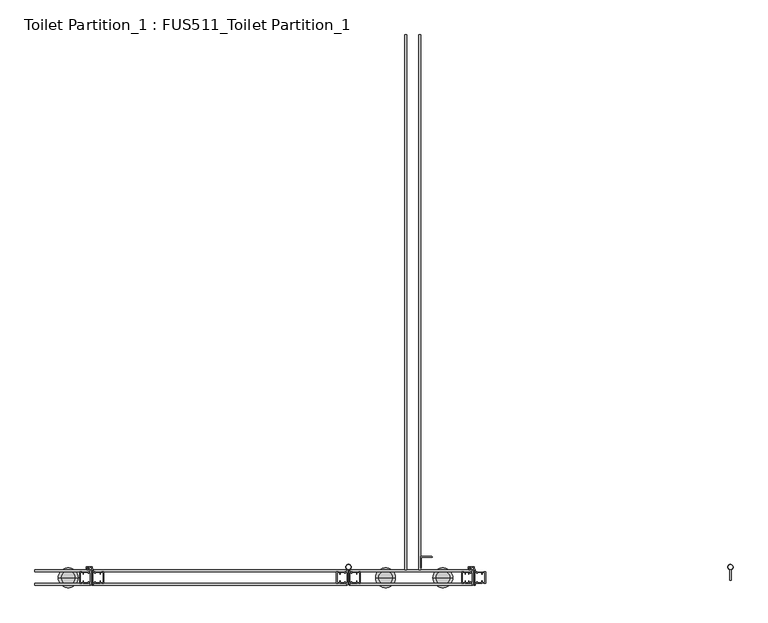
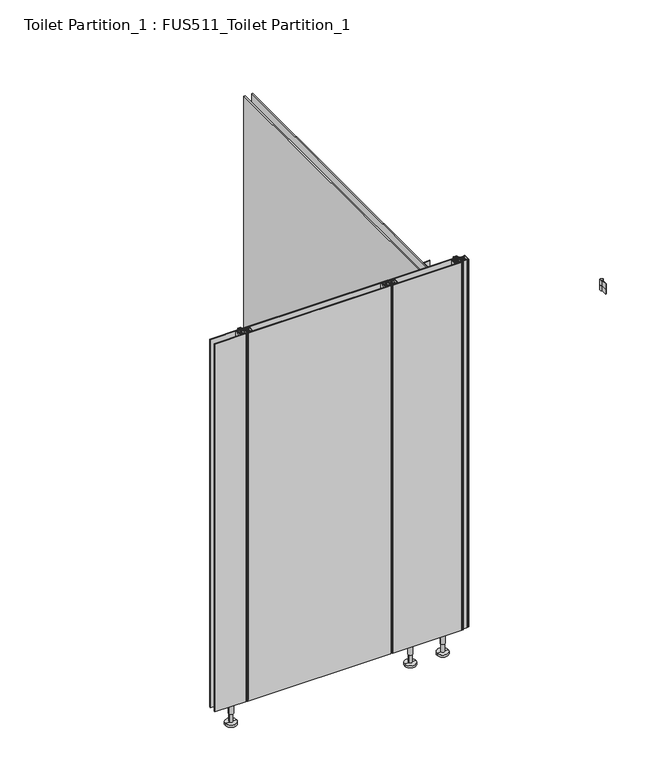
"""IFC4 building model written with IfcOpenShell, lengths in millimetres: furniture geometry, Toilet Partition_1 : FUS511_Toilet Partition_1."""

from ifc_helpers import new_model, si_unit, point, frame, frame_2d, origin, place, context, project, spatial, polyline, circle_curve, trimmed, segment, composite_curve, outline, extrude, source, transform, mapped, element, save
from ifc_brep_helpers import plane_surface, cylinder_surface, advanced_brep


def toilet_partition_1_fus511_toilet_partition_1_6e150948(model_context):
    return source(origin(), model_context, "Body", "SolidModel", [
        extrude(outline(composite_curve([segment(trimmed(circle_curve(frame_2d((-483.6851629, 527.0159753)), 1.0008364), [point((-483.6851629, 528.0168117))], [point((-484.6859993, 527.0159753))], True, "CARTESIAN"), True, "CONTINUOUS"), segment(polyline([(-484.6859993, 527.0159753), (-484.6859993, 499.9933923), (-485.6868357, 499.9933923)]), True, "CONTINUOUS"), segment(trimmed(circle_curve(frame_2d((-485.6868357, 500.9942287)), 1.0008364), [point((-485.6868357, 499.9933923))], [point((-486.6876721, 500.9942287))], False, "CARTESIAN"), True, "CONTINUOUS"), segment(polyline([(-486.6876721, 500.9942287), (-486.6876721, 530.0184846), (-457.6634163, 530.0184846)]), True, "CONTINUOUS"), segment(trimmed(circle_curve(frame_2d((-457.6634163, 529.0176481)), 1.0008364), [point((-457.6634163, 530.0184846))], [point((-456.6625798, 529.0176481))], False, "CARTESIAN"), True, "CONTINUOUS"), segment(polyline([(-456.6625798, 529.0176481), (-456.6625798, 528.0168117), (-483.6851629, 528.0168117)]), True, "CONTINUOUS")], self_intersect=False)), frame((0.0, 0.0, 100.0), z_axis=(0.0, 0.0, 1.0), x_axis=(1.0, 0.0, 0.0)), (0.0, 0.0, 1.0), 1800.0),
        extrude(outline(composite_curve([segment(trimmed(circle_curve(frame_2d((323.7360042, 502.2850056)), 7.0), [point((321.7360042, 495.5768017))], [point((325.7360042, 495.5768017))], False, "CARTESIAN"), True, "CONTINUOUS"), segment(polyline([(325.7360042, 495.5768017), (325.7360042, 467.7850056), (321.7360042, 467.7850056), (321.7360042, 495.5768017)]), True, "CONTINUOUS")], self_intersect=False), holes=[composite_curve([segment(trimmed(circle_curve(frame_2d((323.7360042, 502.2850056)), 6.0), [point((317.7360042, 502.2850056))], [point((329.7360042, 502.2850056))], True, "CARTESIAN"), True, "CONTINUOUS"), segment(trimmed(circle_curve(frame_2d((323.7360042, 502.2850056)), 6.0), [point((329.7360042, 502.2850056))], [point((317.7360042, 502.2850056))], True, "CARTESIAN"), True, "CONTINUOUS")], self_intersect=False)]), frame((0.0, 0.0, 1525.0), z_axis=(0.0, 0.0, 1.0), x_axis=(1.0, 0.0, 0.0)), (0.0, 0.0, 1.0), 25.0),
        extrude(outline(composite_curve([segment(trimmed(circle_curve(frame_2d((323.7360042, 502.2850056)), 7.0), [point((321.7360042, 495.5768017))], [point((325.7360042, 495.5768017))], False, "CARTESIAN"), True, "CONTINUOUS"), segment(polyline([(325.7360042, 495.5768017), (325.7360042, 467.7850056), (321.7360042, 467.7850056), (321.7360042, 495.5768017)]), True, "CONTINUOUS")], self_intersect=False), holes=[composite_curve([segment(trimmed(circle_curve(frame_2d((323.7360042, 502.2850056)), 6.0), [point((317.7360042, 502.2850056))], [point((329.7360042, 502.2850056))], True, "CARTESIAN"), True, "CONTINUOUS"), segment(trimmed(circle_curve(frame_2d((323.7360042, 502.2850056)), 6.0), [point((329.7360042, 502.2850056))], [point((317.7360042, 502.2850056))], True, "CARTESIAN"), True, "CONTINUOUS")], self_intersect=False)]), frame((0.0, 0.0, 1500.0), z_axis=(0.0, 0.0, 1.0), x_axis=(1.0, 0.0, 0.0)), (0.0, 0.0, 1.0), 25.0),
        extrude(outline(composite_curve([segment(trimmed(circle_curve(frame_2d((-675.1953266, 502.2850056)), 7.0), [point((-677.1953266, 495.5768017))], [point((-673.1953266, 495.5768017))], False, "CARTESIAN"), True, "CONTINUOUS"), segment(polyline([(-673.1953266, 495.5768017), (-673.1953266, 467.7850056), (-677.1953266, 467.7850056), (-677.1953266, 495.5768017)]), True, "CONTINUOUS")], self_intersect=False), holes=[composite_curve([segment(trimmed(circle_curve(frame_2d((-675.1953266, 502.2850056)), 6.0), [point((-681.1953266, 502.2850056))], [point((-669.1953266, 502.2850056))], True, "CARTESIAN"), True, "CONTINUOUS"), segment(trimmed(circle_curve(frame_2d((-675.1953266, 502.2850056)), 6.0), [point((-669.1953266, 502.2850056))], [point((-681.1953266, 502.2850056))], True, "CARTESIAN"), True, "CONTINUOUS")], self_intersect=False)]), frame((0.0, 0.0, 1525.0), z_axis=(0.0, 0.0, 1.0), x_axis=(1.0, 0.0, 0.0)), (0.0, 0.0, 1.0), 25.0),
        extrude(outline(composite_curve([segment(trimmed(circle_curve(frame_2d((-675.1953266, 502.2850056)), 7.0), [point((-677.1953266, 495.5768017))], [point((-673.1953266, 495.5768017))], False, "CARTESIAN"), True, "CONTINUOUS"), segment(polyline([(-673.1953266, 495.5768017), (-673.1953266, 467.7850056), (-677.1953266, 467.7850056), (-677.1953266, 495.5768017)]), True, "CONTINUOUS")], self_intersect=False), holes=[composite_curve([segment(trimmed(circle_curve(frame_2d((-675.1953266, 502.2850056)), 6.0), [point((-681.1953266, 502.2850056))], [point((-669.1953266, 502.2850056))], True, "CARTESIAN"), True, "CONTINUOUS"), segment(trimmed(circle_curve(frame_2d((-675.1953266, 502.2850056)), 6.0), [point((-669.1953266, 502.2850056))], [point((-681.1953266, 502.2850056))], True, "CARTESIAN"), True, "CONTINUOUS")], self_intersect=False)]), frame((0.0, 0.0, 1500.0), z_axis=(0.0, 0.0, 1.0), x_axis=(1.0, 0.0, 0.0)), (0.0, 0.0, 1.0), 25.0),
        extrude(outline(composite_curve([segment(trimmed(circle_curve(frame_2d((-675.1953266, 502.2850056)), 7.0), [point((-677.1953266, 495.5768017))], [point((-673.1953266, 495.5768017))], False, "CARTESIAN"), True, "CONTINUOUS"), segment(polyline([(-673.1953266, 495.5768017), (-673.1953266, 467.7850056), (-677.1953266, 467.7850056), (-677.1953266, 495.5768017)]), True, "CONTINUOUS")], self_intersect=False), holes=[composite_curve([segment(trimmed(circle_curve(frame_2d((-675.1953266, 502.2850056)), 6.0), [point((-681.1953266, 502.2850056))], [point((-669.1953266, 502.2850056))], True, "CARTESIAN"), True, "CONTINUOUS"), segment(trimmed(circle_curve(frame_2d((-675.1953266, 502.2850056)), 6.0), [point((-669.1953266, 502.2850056))], [point((-681.1953266, 502.2850056))], True, "CARTESIAN"), True, "CONTINUOUS")], self_intersect=False)]), frame((0.0, 0.0, 525.0), z_axis=(0.0, 0.0, 1.0), x_axis=(1.0, 0.0, 0.0)), (0.0, 0.0, 1.0), 25.0),
        extrude(outline(composite_curve([segment(trimmed(circle_curve(frame_2d((-675.1953266, 502.2850056)), 7.0), [point((-677.1953266, 495.5768017))], [point((-673.1953266, 495.5768017))], False, "CARTESIAN"), True, "CONTINUOUS"), segment(polyline([(-673.1953266, 495.5768017), (-673.1953266, 467.7850056), (-677.1953266, 467.7850056), (-677.1953266, 495.5768017)]), True, "CONTINUOUS")], self_intersect=False), holes=[composite_curve([segment(trimmed(circle_curve(frame_2d((-675.1953266, 502.2850056)), 6.0), [point((-681.1953266, 502.2850056))], [point((-669.1953266, 502.2850056))], True, "CARTESIAN"), True, "CONTINUOUS"), segment(trimmed(circle_curve(frame_2d((-675.1953266, 502.2850056)), 6.0), [point((-669.1953266, 502.2850056))], [point((-681.1953266, 502.2850056))], True, "CARTESIAN"), True, "CONTINUOUS")], self_intersect=False)]), frame((0.0, 0.0, 500.0), z_axis=(0.0, 0.0, 1.0), x_axis=(1.0, 0.0, 0.0)), (0.0, 0.0, 1.0), 25.0),
        extrude(outline(polyline([(-362.0057179, 503.4888254), (-346.2123372, 503.4888254), (-346.2123372, 499.4012527), (-343.7610226, 495.1554513), (-344.9008117, 495.1554513), (-346.2123372, 497.4270801), (-346.2123372, 454.1345106), (-348.1865098, 454.1345106), (-348.1865098, 501.5146528), (-351.8090644, 501.5146528), (-355.8676911, 497.0112968), (-357.0074802, 497.0112968), (-352.9488535, 501.5146528), (-361.0186316, 501.5146528), (-361.0186316, 497.8847941), (-359.6089619, 497.8847941), (-359.6089619, 497.0402783), (-362.0057179, 497.0402783), (-362.0057179, 503.4888254)])), frame((0.0, 0.0, 100.0), z_axis=(0.0, 0.0, 1.0), x_axis=(1.0, 0.0, 0.0)), (0.0, 0.0, 1.0), 1800.0),
        extrude(outline(composite_curve([segment(polyline([(-356.8013826, 495.214347), (-359.8366303, 495.214347)]), True, "CONTINUOUS"), segment(trimmed(circle_curve(frame_2d((-359.8366303, 496.004016)), 0.789669), [point((-359.8366303, 495.214347))], [point((-360.6262994, 496.004016))], False, "CARTESIAN"), True, "CONTINUOUS"), segment(polyline([(-360.6262994, 496.004016), (-360.6262994, 496.8402783), (-359.4784683, 496.8402783)]), True, "CONTINUOUS"), segment(trimmed(circle_curve(frame_2d((-360.1213764, 497.4916495)), 0.9152132), [point((-359.4784683, 496.8402783))], [point((-359.510056, 498.1727534))], True, "CARTESIAN"), True, "CONTINUOUS"), segment(trimmed(circle_curve(frame_2d((-359.2317253, 498.4828563)), 0.4166915), [point((-359.510056, 498.1727534))], [point((-359.3854807, 498.870143))], False, "CARTESIAN"), True, "CONTINUOUS"), segment(trimmed(circle_curve(frame_2d((-358.3136033, 496.1702449)), 2.9048875), [point((-359.3854807, 498.870143))], [point((-357.2177122, 498.8604854))], False, "CARTESIAN"), True, "CONTINUOUS"), segment(trimmed(circle_curve(frame_2d((-357.3679142, 498.4917631)), 0.3981417), [point((-357.2177122, 498.8604854))], [point((-357.1098506, 498.1885801))], False, "CARTESIAN"), True, "CONTINUOUS"), segment(trimmed(circle_curve(frame_2d((-356.5166366, 497.4916495)), 0.9152132), [point((-357.1098506, 498.1885801))], [point((-357.1595447, 496.8402783))], True, "CARTESIAN"), True, "CONTINUOUS"), segment(polyline([(-357.1595447, 496.8402783), (-356.0117136, 496.8402783), (-356.0117136, 496.004016)]), True, "CONTINUOUS"), segment(trimmed(circle_curve(frame_2d((-356.8013826, 496.004016)), 0.789669), [point((-356.0117136, 496.004016))], [point((-356.8013826, 495.214347))], False, "CARTESIAN"), True, "CONTINUOUS")], self_intersect=False)), frame((0.0, 0.0, 100.0), z_axis=(0.0, 0.0, 1.0), x_axis=(1.0, 0.0, 0.0)), (0.0, 0.0, 1.0), 1800.0),
        extrude(outline(polyline([(-1360.9370525, 503.4888254), (-1345.1436718, 503.4888254), (-1345.1436718, 499.4012527), (-1342.6923572, 495.1554513), (-1343.8321463, 495.1554513), (-1345.1436718, 497.4270801), (-1345.1436718, 454.1345106), (-1347.1178444, 454.1345106), (-1347.1178444, 501.5146528), (-1350.740399, 501.5146528), (-1354.7990257, 497.0112968), (-1355.9388148, 497.0112968), (-1351.8801881, 501.5146528), (-1359.9499662, 501.5146528), (-1359.9499662, 497.8847941), (-1358.5402965, 497.8847941), (-1358.5402965, 497.0402783), (-1360.9370525, 497.0402783), (-1360.9370525, 503.4888254)])), frame((0.0, 0.0, 100.0), z_axis=(0.0, 0.0, 1.0), x_axis=(1.0, 0.0, 0.0)), (0.0, 0.0, 1.0), 1800.0),
        extrude(outline(composite_curve([segment(polyline([(-1355.7327172, 495.214347), (-1358.7679649, 495.214347)]), True, "CONTINUOUS"), segment(trimmed(circle_curve(frame_2d((-1358.7679649, 496.004016)), 0.789669), [point((-1358.7679649, 495.214347))], [point((-1359.557634, 496.004016))], False, "CARTESIAN"), True, "CONTINUOUS"), segment(polyline([(-1359.557634, 496.004016), (-1359.557634, 496.8402783), (-1358.4098029, 496.8402783)]), True, "CONTINUOUS"), segment(trimmed(circle_curve(frame_2d((-1359.052711, 497.4916495)), 0.9152132), [point((-1358.4098029, 496.8402783))], [point((-1358.4413906, 498.1727534))], True, "CARTESIAN"), True, "CONTINUOUS"), segment(trimmed(circle_curve(frame_2d((-1358.1630599, 498.4828563)), 0.4166915), [point((-1358.4413906, 498.1727534))], [point((-1358.3168153, 498.870143))], False, "CARTESIAN"), True, "CONTINUOUS"), segment(trimmed(circle_curve(frame_2d((-1357.2449378, 496.1702449)), 2.9048875), [point((-1358.3168153, 498.870143))], [point((-1356.1490468, 498.8604854))], False, "CARTESIAN"), True, "CONTINUOUS"), segment(trimmed(circle_curve(frame_2d((-1356.2992488, 498.4917631)), 0.3981417), [point((-1356.1490468, 498.8604854))], [point((-1356.0411852, 498.1885801))], False, "CARTESIAN"), True, "CONTINUOUS"), segment(trimmed(circle_curve(frame_2d((-1355.4479712, 497.4916495)), 0.9152132), [point((-1356.0411852, 498.1885801))], [point((-1356.0908793, 496.8402783))], True, "CARTESIAN"), True, "CONTINUOUS"), segment(polyline([(-1356.0908793, 496.8402783), (-1354.9430482, 496.8402783), (-1354.9430482, 496.004016)]), True, "CONTINUOUS"), segment(trimmed(circle_curve(frame_2d((-1355.7327172, 496.004016)), 0.789669), [point((-1354.9430482, 496.004016))], [point((-1355.7327172, 495.214347))], False, "CARTESIAN"), True, "CONTINUOUS")], self_intersect=False)), frame((0.0, 0.0, 100.0), z_axis=(0.0, 0.0, 1.0), x_axis=(1.0, 0.0, 0.0)), (0.0, 0.0, 1.0), 1800.0),
        advanced_brep(
        [(-443.912605, 474.714347, 104.1461397), (-412.6687631, 474.714347, 104.1461397), (-412.6687631, 474.714347, 101.0217555), (-443.912605, 474.714347, 101.0217555), (-454.3272189, 474.714347, 0.0), (-402.2541491, 474.714347, 0.0), (-428.290684, 474.714347, 0.0), (-454.3272189, 474.714347, 10.414614), (-402.2541491, 474.714347, 10.414614), (-436.1016445, 474.714347, 10.414614), (-420.4797235, 474.714347, 10.414614), (-436.1016445, 474.714347, 52.0730698), (-420.4797235, 474.714347, 52.0730698), (-438.705298, 474.714347, 52.0730698), (-417.8760701, 474.714347, 52.0730698), (-438.705298, 474.714347, 101.0217555), (-417.8760701, 474.714347, 101.0217555), (-445.9955278, 474.714347, 104.1461397), (-410.5858403, 474.714347, 104.1461397), (-445.9955278, 474.714347, 110.394908), (-410.5858403, 474.714347, 110.394908), (-428.290684, 474.714347, 110.394908)],
        [
            (0, 1, circle_curve(frame((-428.290684, 474.714347, 104.1461397), z_axis=(0.0, 0.0, -1.0), x_axis=(1.0, 0.0, 0.0)), 15.6219209)),
            (1, 2),
            (2, 3, circle_curve(frame((-428.290684, 474.714347, 101.0217555), z_axis=(0.0, 0.0, 1.0), x_axis=(1.0, 0.0, 0.0)), 15.6219209)),
            (3, 0),
            (1, 0, circle_curve(frame((-428.290684, 474.714347, 104.1461397), z_axis=(0.0, 0.0, -1.0), x_axis=(1.0, 0.0, 0.0)), 15.6219209)),
            (3, 2, circle_curve(frame((-428.290684, 474.714347, 101.0217555), z_axis=(0.0, 0.0, 1.0), x_axis=(1.0, 0.0, 0.0)), 15.6219209)),
            (4, 5, circle_curve(frame((-428.290684, 474.714347, 0.0), z_axis=(0.0, 0.0, -1.0), x_axis=(1.0, 0.0, 0.0)), 26.0365349)),
            (5, 6),
            (6, 4),
            (5, 4, circle_curve(frame((-428.290684, 474.714347, 0.0), z_axis=(0.0, 0.0, -1.0), x_axis=(1.0, 0.0, 0.0)), 26.0365349)),
            (7, 8, circle_curve(frame((-428.290684, 474.714347, 10.414614), z_axis=(0.0, 0.0, -1.0), x_axis=(1.0, 0.0, 0.0)), 26.0365349)),
            (8, 5),
            (4, 7),
            (8, 7, circle_curve(frame((-428.290684, 474.714347, 10.414614), z_axis=(0.0, 0.0, -1.0), x_axis=(1.0, 0.0, 0.0)), 26.0365349)),
            (9, 10, circle_curve(frame((-428.290684, 474.714347, 10.414614), z_axis=(0.0, 0.0, -1.0), x_axis=(1.0, 0.0, 0.0)), 7.8109605)),
            (10, 8),
            (7, 9),
            (10, 9, circle_curve(frame((-428.290684, 474.714347, 10.414614), z_axis=(0.0, 0.0, -1.0), x_axis=(1.0, 0.0, 0.0)), 7.8109605)),
            (11, 12, circle_curve(frame((-428.290684, 474.714347, 52.0730698), z_axis=(0.0, 0.0, -1.0), x_axis=(1.0, 0.0, 0.0)), 7.8109605)),
            (12, 10),
            (9, 11),
            (12, 11, circle_curve(frame((-428.290684, 474.714347, 52.0730698), z_axis=(0.0, 0.0, -1.0), x_axis=(1.0, 0.0, 0.0)), 7.8109605)),
            (13, 14, circle_curve(frame((-428.290684, 474.714347, 52.0730698), z_axis=(0.0, 0.0, -1.0), x_axis=(1.0, 0.0, 0.0)), 10.414614)),
            (14, 12),
            (11, 13),
            (14, 13, circle_curve(frame((-428.290684, 474.714347, 52.0730698), z_axis=(0.0, 0.0, -1.0), x_axis=(1.0, 0.0, 0.0)), 10.414614)),
            (15, 16, circle_curve(frame((-428.290684, 474.714347, 101.0217555), z_axis=(0.0, 0.0, -1.0), x_axis=(1.0, 0.0, 0.0)), 10.414614)),
            (16, 14),
            (13, 15),
            (16, 15, circle_curve(frame((-428.290684, 474.714347, 101.0217555), z_axis=(0.0, 0.0, -1.0), x_axis=(1.0, 0.0, 0.0)), 10.414614)),
            (2, 16),
            (15, 3),
            (17, 18, circle_curve(frame((-428.290684, 474.714347, 104.1461397), z_axis=(0.0, 0.0, -1.0), x_axis=(1.0, 0.0, 0.0)), 17.7048437)),
            (18, 1),
            (0, 17),
            (18, 17, circle_curve(frame((-428.290684, 474.714347, 104.1461397), z_axis=(0.0, 0.0, -1.0), x_axis=(1.0, 0.0, 0.0)), 17.7048437)),
            (19, 20, circle_curve(frame((-428.290684, 474.714347, 110.394908), z_axis=(0.0, 0.0, -1.0), x_axis=(1.0, 0.0, 0.0)), 17.7048437)),
            (20, 18),
            (17, 19),
            (20, 19, circle_curve(frame((-428.290684, 474.714347, 110.394908), z_axis=(0.0, 0.0, -1.0), x_axis=(1.0, 0.0, 0.0)), 17.7048437)),
            (21, 20),
            (19, 21),
        ],
        [
            cylinder_surface(frame((-428.290684, 474.714347, 190.0), z_axis=(0.0, 0.0, 1.0), x_axis=(1.0, 0.0, 0.0)), 15.6219209),
            plane_surface(frame((-428.290684, 474.714347, 0.0), z_axis=(0.0, 0.0, -1.0), x_axis=(1.0, 0.0, 0.0))),
            cylinder_surface(frame((-428.290684, 474.714347, 190.0), z_axis=(0.0, 0.0, 1.0), x_axis=(1.0, 0.0, 0.0)), 26.0365349),
            plane_surface(frame((-428.290684, 474.714347, 10.414614), z_axis=(0.0, 0.0, 1.0), x_axis=(1.0, 0.0, 0.0))),
            cylinder_surface(frame((-428.290684, 474.714347, 190.0), z_axis=(0.0, 0.0, 1.0), x_axis=(1.0, 0.0, 0.0)), 7.8109605),
            plane_surface(frame((-428.290684, 474.714347, 52.0730698), z_axis=(0.0, 0.0, -1.0), x_axis=(1.0, 0.0, 0.0))),
            cylinder_surface(frame((-428.290684, 474.714347, 190.0), z_axis=(0.0, 0.0, 1.0), x_axis=(1.0, 0.0, 0.0)), 10.414614),
            plane_surface(frame((-428.290684, 474.714347, 101.0217555), z_axis=(0.0, 0.0, -1.0), x_axis=(1.0, 0.0, 0.0))),
            plane_surface(frame((-428.290684, 474.714347, 104.1461397), z_axis=(0.0, 0.0, -1.0), x_axis=(1.0, 0.0, 0.0))),
            cylinder_surface(frame((-428.290684, 474.714347, 190.0), z_axis=(0.0, 0.0, 1.0), x_axis=(1.0, 0.0, 0.0)), 17.7048437),
            plane_surface(frame((-428.290684, 474.714347, 110.394908), z_axis=(0.0, 0.0, 1.0), x_axis=(1.0, 0.0, 0.0))),
        ],
        [
            (0, [[1, 2, 3, 4]]),
            (0, [[5, -4, 6, -2]]),
            (1, [[7, 8, 9]]),
            (1, [[10, -9, -8]]),
            (2, [[11, 12, -7, 13]]),
            (2, [[14, -13, -10, -12]]),
            (3, [[15, 16, -11, 17]]),
            (3, [[18, -17, -14, -16]]),
            (4, [[19, 20, -15, 21]]),
            (4, [[22, -21, -18, -20]]),
            (5, [[23, 24, -19, 25]]),
            (5, [[26, -25, -22, -24]]),
            (6, [[27, 28, -23, 29]]),
            (6, [[30, -29, -26, -28]]),
            (7, [[-3, 31, -27, 32]]),
            (7, [[-6, -32, -30, -31]]),
            (8, [[33, 34, -1, 35]]),
            (8, [[36, -35, -5, -34]]),
            (9, [[37, 38, -33, 39]]),
            (9, [[40, -39, -36, -38]]),
            (10, [[41, -37, 42]]),
            (10, [[-42, -40, -41]]),
        ],
    ),
        advanced_brep(
        [(-593.912605, 474.714347, 104.1461397), (-562.6687631, 474.714347, 104.1461397), (-562.6687631, 474.714347, 101.0217555), (-593.912605, 474.714347, 101.0217555), (-604.3272189, 474.714347, 0.0), (-552.2541491, 474.714347, 0.0), (-578.290684, 474.714347, 0.0), (-604.3272189, 474.714347, 10.414614), (-552.2541491, 474.714347, 10.414614), (-586.1016445, 474.714347, 10.414614), (-570.4797235, 474.714347, 10.414614), (-586.1016445, 474.714347, 52.0730698), (-570.4797235, 474.714347, 52.0730698), (-588.705298, 474.714347, 52.0730698), (-567.8760701, 474.714347, 52.0730698), (-588.705298, 474.714347, 101.0217555), (-567.8760701, 474.714347, 101.0217555), (-595.9955278, 474.714347, 104.1461397), (-560.5858403, 474.714347, 104.1461397), (-595.9955278, 474.714347, 110.394908), (-560.5858403, 474.714347, 110.394908), (-578.290684, 474.714347, 110.394908)],
        [
            (0, 1, circle_curve(frame((-578.290684, 474.714347, 104.1461397), z_axis=(0.0, 0.0, -1.0), x_axis=(1.0, 0.0, 0.0)), 15.6219209)),
            (1, 2),
            (2, 3, circle_curve(frame((-578.290684, 474.714347, 101.0217555), z_axis=(0.0, 0.0, 1.0), x_axis=(1.0, 0.0, 0.0)), 15.6219209)),
            (3, 0),
            (1, 0, circle_curve(frame((-578.290684, 474.714347, 104.1461397), z_axis=(0.0, 0.0, -1.0), x_axis=(1.0, 0.0, 0.0)), 15.6219209)),
            (3, 2, circle_curve(frame((-578.290684, 474.714347, 101.0217555), z_axis=(0.0, 0.0, 1.0), x_axis=(1.0, 0.0, 0.0)), 15.6219209)),
            (4, 5, circle_curve(frame((-578.290684, 474.714347, 0.0), z_axis=(0.0, 0.0, -1.0), x_axis=(1.0, 0.0, 0.0)), 26.0365349)),
            (5, 6),
            (6, 4),
            (5, 4, circle_curve(frame((-578.290684, 474.714347, 0.0), z_axis=(0.0, 0.0, -1.0), x_axis=(1.0, 0.0, 0.0)), 26.0365349)),
            (7, 8, circle_curve(frame((-578.290684, 474.714347, 10.414614), z_axis=(0.0, 0.0, -1.0), x_axis=(1.0, 0.0, 0.0)), 26.0365349)),
            (8, 5),
            (4, 7),
            (8, 7, circle_curve(frame((-578.290684, 474.714347, 10.414614), z_axis=(0.0, 0.0, -1.0), x_axis=(1.0, 0.0, 0.0)), 26.0365349)),
            (9, 10, circle_curve(frame((-578.290684, 474.714347, 10.414614), z_axis=(0.0, 0.0, -1.0), x_axis=(1.0, 0.0, 0.0)), 7.8109605)),
            (10, 8),
            (7, 9),
            (10, 9, circle_curve(frame((-578.290684, 474.714347, 10.414614), z_axis=(0.0, 0.0, -1.0), x_axis=(1.0, 0.0, 0.0)), 7.8109605)),
            (11, 12, circle_curve(frame((-578.290684, 474.714347, 52.0730698), z_axis=(0.0, 0.0, -1.0), x_axis=(1.0, 0.0, 0.0)), 7.8109605)),
            (12, 10),
            (9, 11),
            (12, 11, circle_curve(frame((-578.290684, 474.714347, 52.0730698), z_axis=(0.0, 0.0, -1.0), x_axis=(1.0, 0.0, 0.0)), 7.8109605)),
            (13, 14, circle_curve(frame((-578.290684, 474.714347, 52.0730698), z_axis=(0.0, 0.0, -1.0), x_axis=(1.0, 0.0, 0.0)), 10.414614)),
            (14, 12),
            (11, 13),
            (14, 13, circle_curve(frame((-578.290684, 474.714347, 52.0730698), z_axis=(0.0, 0.0, -1.0), x_axis=(1.0, 0.0, 0.0)), 10.414614)),
            (15, 16, circle_curve(frame((-578.290684, 474.714347, 101.0217555), z_axis=(0.0, 0.0, -1.0), x_axis=(1.0, 0.0, 0.0)), 10.414614)),
            (16, 14),
            (13, 15),
            (16, 15, circle_curve(frame((-578.290684, 474.714347, 101.0217555), z_axis=(0.0, 0.0, -1.0), x_axis=(1.0, 0.0, 0.0)), 10.414614)),
            (2, 16),
            (15, 3),
            (17, 18, circle_curve(frame((-578.290684, 474.714347, 104.1461397), z_axis=(0.0, 0.0, -1.0), x_axis=(1.0, 0.0, 0.0)), 17.7048437)),
            (18, 1),
            (0, 17),
            (18, 17, circle_curve(frame((-578.290684, 474.714347, 104.1461397), z_axis=(0.0, 0.0, -1.0), x_axis=(1.0, 0.0, 0.0)), 17.7048437)),
            (19, 20, circle_curve(frame((-578.290684, 474.714347, 110.394908), z_axis=(0.0, 0.0, -1.0), x_axis=(1.0, 0.0, 0.0)), 17.7048437)),
            (20, 18),
            (17, 19),
            (20, 19, circle_curve(frame((-578.290684, 474.714347, 110.394908), z_axis=(0.0, 0.0, -1.0), x_axis=(1.0, 0.0, 0.0)), 17.7048437)),
            (21, 20),
            (19, 21),
        ],
        [
            cylinder_surface(frame((-578.290684, 474.714347, 190.0), z_axis=(0.0, 0.0, 1.0), x_axis=(1.0, 0.0, 0.0)), 15.6219209),
            plane_surface(frame((-578.290684, 474.714347, 0.0), z_axis=(0.0, 0.0, -1.0), x_axis=(1.0, 0.0, 0.0))),
            cylinder_surface(frame((-578.290684, 474.714347, 190.0), z_axis=(0.0, 0.0, 1.0), x_axis=(1.0, 0.0, 0.0)), 26.0365349),
            plane_surface(frame((-578.290684, 474.714347, 10.414614), z_axis=(0.0, 0.0, 1.0), x_axis=(1.0, 0.0, 0.0))),
            cylinder_surface(frame((-578.290684, 474.714347, 190.0), z_axis=(0.0, 0.0, 1.0), x_axis=(1.0, 0.0, 0.0)), 7.8109605),
            plane_surface(frame((-578.290684, 474.714347, 52.0730698), z_axis=(0.0, 0.0, -1.0), x_axis=(1.0, 0.0, 0.0))),
            cylinder_surface(frame((-578.290684, 474.714347, 190.0), z_axis=(0.0, 0.0, 1.0), x_axis=(1.0, 0.0, 0.0)), 10.414614),
            plane_surface(frame((-578.290684, 474.714347, 101.0217555), z_axis=(0.0, 0.0, -1.0), x_axis=(1.0, 0.0, 0.0))),
            plane_surface(frame((-578.290684, 474.714347, 104.1461397), z_axis=(0.0, 0.0, -1.0), x_axis=(1.0, 0.0, 0.0))),
            cylinder_surface(frame((-578.290684, 474.714347, 190.0), z_axis=(0.0, 0.0, 1.0), x_axis=(1.0, 0.0, 0.0)), 17.7048437),
            plane_surface(frame((-578.290684, 474.714347, 110.394908), z_axis=(0.0, 0.0, 1.0), x_axis=(1.0, 0.0, 0.0))),
        ],
        [
            (0, [[1, 2, 3, 4]]),
            (0, [[5, -4, 6, -2]]),
            (1, [[7, 8, 9]]),
            (1, [[10, -9, -8]]),
            (2, [[11, 12, -7, 13]]),
            (2, [[14, -13, -10, -12]]),
            (3, [[15, 16, -11, 17]]),
            (3, [[18, -17, -14, -16]]),
            (4, [[19, 20, -15, 21]]),
            (4, [[22, -21, -18, -20]]),
            (5, [[23, 24, -19, 25]]),
            (5, [[26, -25, -22, -24]]),
            (6, [[27, 28, -23, 29]]),
            (6, [[30, -29, -26, -28]]),
            (7, [[-3, 31, -27, 32]]),
            (7, [[-6, -32, -30, -31]]),
            (8, [[33, 34, -1, 35]]),
            (8, [[36, -35, -5, -34]]),
            (9, [[37, 38, -33, 39]]),
            (9, [[40, -39, -36, -38]]),
            (10, [[41, -37, 42]]),
            (10, [[-42, -40, -41]]),
        ],
    ),
        advanced_brep(
        [(-1423.912605, 474.714347, 104.1461397), (-1392.6687631, 474.714347, 104.1461397), (-1392.6687631, 474.714347, 101.0217555), (-1423.912605, 474.714347, 101.0217555), (-1434.3272189, 474.714347, 0.0), (-1382.2541491, 474.714347, 0.0), (-1408.290684, 474.714347, 0.0), (-1434.3272189, 474.714347, 10.414614), (-1382.2541491, 474.714347, 10.414614), (-1416.1016445, 474.714347, 10.414614), (-1400.4797235, 474.714347, 10.414614), (-1416.1016445, 474.714347, 52.0730698), (-1400.4797235, 474.714347, 52.0730698), (-1418.705298, 474.714347, 52.0730698), (-1397.8760701, 474.714347, 52.0730698), (-1418.705298, 474.714347, 101.0217555), (-1397.8760701, 474.714347, 101.0217555), (-1425.9955278, 474.714347, 104.1461397), (-1390.5858403, 474.714347, 104.1461397), (-1425.9955278, 474.714347, 110.394908), (-1390.5858403, 474.714347, 110.394908), (-1408.290684, 474.714347, 110.394908)],
        [
            (0, 1, circle_curve(frame((-1408.290684, 474.714347, 104.1461397), z_axis=(0.0, 0.0, -1.0), x_axis=(1.0, 0.0, 0.0)), 15.6219209)),
            (1, 2),
            (2, 3, circle_curve(frame((-1408.290684, 474.714347, 101.0217555), z_axis=(0.0, 0.0, 1.0), x_axis=(1.0, 0.0, 0.0)), 15.6219209)),
            (3, 0),
            (1, 0, circle_curve(frame((-1408.290684, 474.714347, 104.1461397), z_axis=(0.0, 0.0, -1.0), x_axis=(1.0, 0.0, 0.0)), 15.6219209)),
            (3, 2, circle_curve(frame((-1408.290684, 474.714347, 101.0217555), z_axis=(0.0, 0.0, 1.0), x_axis=(1.0, 0.0, 0.0)), 15.6219209)),
            (4, 5, circle_curve(frame((-1408.290684, 474.714347, 0.0), z_axis=(0.0, 0.0, -1.0), x_axis=(1.0, 0.0, 0.0)), 26.0365349)),
            (5, 6),
            (6, 4),
            (5, 4, circle_curve(frame((-1408.290684, 474.714347, 0.0), z_axis=(0.0, 0.0, -1.0), x_axis=(1.0, 0.0, 0.0)), 26.0365349)),
            (7, 8, circle_curve(frame((-1408.290684, 474.714347, 10.414614), z_axis=(0.0, 0.0, -1.0), x_axis=(1.0, 0.0, 0.0)), 26.0365349)),
            (8, 5),
            (4, 7),
            (8, 7, circle_curve(frame((-1408.290684, 474.714347, 10.414614), z_axis=(0.0, 0.0, -1.0), x_axis=(1.0, 0.0, 0.0)), 26.0365349)),
            (9, 10, circle_curve(frame((-1408.290684, 474.714347, 10.414614), z_axis=(0.0, 0.0, -1.0), x_axis=(1.0, 0.0, 0.0)), 7.8109605)),
            (10, 8),
            (7, 9),
            (10, 9, circle_curve(frame((-1408.290684, 474.714347, 10.414614), z_axis=(0.0, 0.0, -1.0), x_axis=(1.0, 0.0, 0.0)), 7.8109605)),
            (11, 12, circle_curve(frame((-1408.290684, 474.714347, 52.0730698), z_axis=(0.0, 0.0, -1.0), x_axis=(1.0, 0.0, 0.0)), 7.8109605)),
            (12, 10),
            (9, 11),
            (12, 11, circle_curve(frame((-1408.290684, 474.714347, 52.0730698), z_axis=(0.0, 0.0, -1.0), x_axis=(1.0, 0.0, 0.0)), 7.8109605)),
            (13, 14, circle_curve(frame((-1408.290684, 474.714347, 52.0730698), z_axis=(0.0, 0.0, -1.0), x_axis=(1.0, 0.0, 0.0)), 10.414614)),
            (14, 12),
            (11, 13),
            (14, 13, circle_curve(frame((-1408.290684, 474.714347, 52.0730698), z_axis=(0.0, 0.0, -1.0), x_axis=(1.0, 0.0, 0.0)), 10.414614)),
            (15, 16, circle_curve(frame((-1408.290684, 474.714347, 101.0217555), z_axis=(0.0, 0.0, -1.0), x_axis=(1.0, 0.0, 0.0)), 10.414614)),
            (16, 14),
            (13, 15),
            (16, 15, circle_curve(frame((-1408.290684, 474.714347, 101.0217555), z_axis=(0.0, 0.0, -1.0), x_axis=(1.0, 0.0, 0.0)), 10.414614)),
            (2, 16),
            (15, 3),
            (17, 18, circle_curve(frame((-1408.290684, 474.714347, 104.1461397), z_axis=(0.0, 0.0, -1.0), x_axis=(1.0, 0.0, 0.0)), 17.7048437)),
            (18, 1),
            (0, 17),
            (18, 17, circle_curve(frame((-1408.290684, 474.714347, 104.1461397), z_axis=(0.0, 0.0, -1.0), x_axis=(1.0, 0.0, 0.0)), 17.7048437)),
            (19, 20, circle_curve(frame((-1408.290684, 474.714347, 110.394908), z_axis=(0.0, 0.0, -1.0), x_axis=(1.0, 0.0, 0.0)), 17.7048437)),
            (20, 18),
            (17, 19),
            (20, 19, circle_curve(frame((-1408.290684, 474.714347, 110.394908), z_axis=(0.0, 0.0, -1.0), x_axis=(1.0, 0.0, 0.0)), 17.7048437)),
            (21, 20),
            (19, 21),
        ],
        [
            cylinder_surface(frame((-1408.290684, 474.714347, 190.0), z_axis=(0.0, 0.0, 1.0), x_axis=(1.0, 0.0, 0.0)), 15.6219209),
            plane_surface(frame((-1408.290684, 474.714347, 0.0), z_axis=(0.0, 0.0, -1.0), x_axis=(1.0, 0.0, 0.0))),
            cylinder_surface(frame((-1408.290684, 474.714347, 190.0), z_axis=(0.0, 0.0, 1.0), x_axis=(1.0, 0.0, 0.0)), 26.0365349),
            plane_surface(frame((-1408.290684, 474.714347, 10.414614), z_axis=(0.0, 0.0, 1.0), x_axis=(1.0, 0.0, 0.0))),
            cylinder_surface(frame((-1408.290684, 474.714347, 190.0), z_axis=(0.0, 0.0, 1.0), x_axis=(1.0, 0.0, 0.0)), 7.8109605),
            plane_surface(frame((-1408.290684, 474.714347, 52.0730698), z_axis=(0.0, 0.0, -1.0), x_axis=(1.0, 0.0, 0.0))),
            cylinder_surface(frame((-1408.290684, 474.714347, 190.0), z_axis=(0.0, 0.0, 1.0), x_axis=(1.0, 0.0, 0.0)), 10.414614),
            plane_surface(frame((-1408.290684, 474.714347, 101.0217555), z_axis=(0.0, 0.0, -1.0), x_axis=(1.0, 0.0, 0.0))),
            plane_surface(frame((-1408.290684, 474.714347, 104.1461397), z_axis=(0.0, 0.0, -1.0), x_axis=(1.0, 0.0, 0.0))),
            cylinder_surface(frame((-1408.290684, 474.714347, 190.0), z_axis=(0.0, 0.0, 1.0), x_axis=(1.0, 0.0, 0.0)), 17.7048437),
            plane_surface(frame((-1408.290684, 474.714347, 110.394908), z_axis=(0.0, 0.0, 1.0), x_axis=(1.0, 0.0, 0.0))),
        ],
        [
            (0, [[1, 2, 3, 4]]),
            (0, [[5, -4, 6, -2]]),
            (1, [[7, 8, 9]]),
            (1, [[10, -9, -8]]),
            (2, [[11, 12, -7, 13]]),
            (2, [[14, -13, -10, -12]]),
            (3, [[15, 16, -11, 17]]),
            (3, [[18, -17, -14, -16]]),
            (4, [[19, 20, -15, 21]]),
            (4, [[22, -21, -18, -20]]),
            (5, [[23, 24, -19, 25]]),
            (5, [[26, -25, -22, -24]]),
            (6, [[27, 28, -23, 29]]),
            (6, [[30, -29, -26, -28]]),
            (7, [[-3, 31, -27, 32]]),
            (7, [[-6, -32, -30, -31]]),
            (8, [[33, 34, -1, 35]]),
            (8, [[36, -35, -5, -34]]),
            (9, [[37, 38, -33, 39]]),
            (9, [[40, -39, -36, -38]]),
            (10, [[41, -37, 42]]),
            (10, [[-42, -40, -41]]),
        ],
    ),
        extrude(outline(polyline([(-486.6876721, 495.214347), (-491.6876721, 495.214347), (-491.6876721, 1895.214347), (-486.6876721, 1895.214347), (-486.6876721, 495.214347)])), frame((0.0, 0.0, 100.0), z_axis=(0.0, 0.0, 1.0), x_axis=(1.0, 0.0, 0.0)), (0.0, 0.0, 1.0), 1800.0),
        extrude(outline(polyline([(-522.6876721, 495.214347), (-527.6876721, 495.214347), (-527.6876721, 1895.214347), (-522.6876721, 1895.214347), (-522.6876721, 495.214347)])), frame((0.0, 0.0, 100.0), z_axis=(0.0, 0.0, 1.0), x_axis=(1.0, 0.0, 0.0)), (0.0, 0.0, 1.0), 1800.0),
        extrude(outline(composite_curve([segment(polyline([(-1378.0265961, 489.5206414), (-1373.0911646, 489.5206414), (-1373.0911646, 488.5335551), (-1369.1428194, 488.5335551), (-1355.5703828, 489.5206414)]), True, "CONTINUOUS"), segment(trimmed(circle_curve(frame_2d((-1355.3236113, 488.5648992)), 0.9870863), [point((-1355.5703828, 489.5206414))], [point((-1355.0768397, 489.5206414))], True, "CARTESIAN"), True, "CONTINUOUS"), segment(polyline([(-1355.0768397, 489.5206414), (-1350.3881798, 489.5206414), (-1350.3881798, 494.4560729), (-1349.4010935, 494.4560729)]), True, "CONTINUOUS"), segment(trimmed(circle_curve(frame_2d((-1349.4010935, 493.4689866)), 0.9870863), [point((-1349.4010935, 494.4560729))], [point((-1348.4140072, 493.4689866))], False, "CARTESIAN"), True, "CONTINUOUS"), segment(polyline([(-1348.4140072, 493.4689866), (-1348.4140072, 455.9597074)]), True, "CONTINUOUS"), segment(trimmed(circle_curve(frame_2d((-1349.4010935, 455.9597074)), 0.9870863), [point((-1348.4140072, 455.9597074))], [point((-1349.4010935, 454.9726211))], False, "CARTESIAN"), True, "CONTINUOUS"), segment(polyline([(-1349.4010935, 454.9726211), (-1350.3881798, 454.9726211), (-1350.3881798, 459.9080525), (-1355.0768397, 459.9080525)]), True, "CONTINUOUS"), segment(trimmed(circle_curve(frame_2d((-1355.3236113, 460.8637947)), 0.9870863), [point((-1355.0768397, 459.9080525))], [point((-1355.5703828, 459.9080525))], True, "CARTESIAN"), True, "CONTINUOUS"), segment(polyline([(-1355.5703828, 459.9080525), (-1369.1428194, 459.9080525), (-1369.1428194, 460.8951388), (-1373.0911646, 460.8951388), (-1373.0911646, 459.9080525), (-1378.0265961, 459.9080525), (-1378.0265961, 489.5206414)]), True, "CONTINUOUS")], self_intersect=False), holes=[polyline([(-1375.0653372, 486.5593825), (-1375.0653372, 462.8693114), (-1370.1299057, 462.8693114), (-1370.1299057, 467.8047429), (-1367.1686468, 467.8047429), (-1367.1686468, 462.8693114), (-1360.2590427, 462.8693114), (-1360.2590427, 467.3111998), (-1358.7784133, 467.3111998), (-1358.7784133, 462.8693114), (-1357.0510123, 462.8693114), (-1357.0510123, 464.843484), (-1353.1026671, 464.843484), (-1353.1026671, 462.8693114), (-1351.3752661, 462.8693114), (-1351.3752661, 486.5593825), (-1353.1026671, 486.5593825), (-1353.1026671, 484.5852099), (-1357.0510123, 484.5852099), (-1357.0510123, 486.5593825), (-1358.7784133, 486.5593825), (-1358.7784133, 482.1174942), (-1360.2590427, 482.1174942), (-1360.2590427, 486.5593825), (-1367.1686468, 486.5593825), (-1367.1686468, 481.623951), (-1370.1299057, 481.623951), (-1370.1299057, 486.5593825), (-1375.0653372, 486.5593825)])]), frame((0.0, 0.0, 100.0), z_axis=(0.0, 0.0, 1.0), x_axis=(1.0, 0.0, 0.0)), (0.0, 0.0, 1.0), 1800.0),
        extrude(outline(polyline([(-1495.3881798, 454.214347), (-1495.3881798, 459.214347), (-1350.3881798, 459.214347), (-1350.3881798, 454.214347), (-1495.3881798, 454.214347)])), frame((0.0, 0.0, 100.0), z_axis=(0.0, 0.0, 1.0), x_axis=(1.0, 0.0, 0.0)), (0.0, 0.0, 1.0), 1800.0),
        extrude(outline(polyline([(-1495.3881798, 490.214347), (-1495.3881798, 495.214347), (-1350.3881798, 495.214347), (-1350.3881798, 490.214347), (-1495.3881798, 490.214347)])), frame((0.0, 0.0, 100.0), z_axis=(0.0, 0.0, 1.0), x_axis=(1.0, 0.0, 0.0)), (0.0, 0.0, 1.0), 1800.0),
        extrude(outline(composite_curve([segment(polyline([(-1315.5310829, 489.5206414), (-1315.5310829, 459.9080525), (-1320.4665144, 459.9080525), (-1320.4665144, 460.8951388), (-1324.4148596, 460.8951388), (-1324.4148596, 459.9080525), (-1337.9872961, 459.9080525)]), True, "CONTINUOUS"), segment(trimmed(circle_curve(frame_2d((-1338.2340677, 460.8637947)), 0.9870863), [point((-1337.9872961, 459.9080525))], [point((-1338.4808393, 459.9080525))], True, "CARTESIAN"), True, "CONTINUOUS"), segment(polyline([(-1338.4808393, 459.9080525), (-1343.1694992, 459.9080525), (-1343.1694992, 454.9726211), (-1344.1565855, 454.9726211)]), True, "CONTINUOUS"), segment(trimmed(circle_curve(frame_2d((-1344.1565855, 455.9597074)), 0.9870863), [point((-1344.1565855, 454.9726211))], [point((-1345.1436718, 455.9597074))], False, "CARTESIAN"), True, "CONTINUOUS"), segment(polyline([(-1345.1436718, 455.9597074), (-1345.1436718, 493.4689866)]), True, "CONTINUOUS"), segment(trimmed(circle_curve(frame_2d((-1344.1565855, 493.4689866)), 0.9870863), [point((-1345.1436718, 493.4689866))], [point((-1344.1565855, 494.4560729))], False, "CARTESIAN"), True, "CONTINUOUS"), segment(polyline([(-1344.1565855, 494.4560729), (-1343.1694992, 494.4560729), (-1343.1694992, 489.5206414), (-1338.4808393, 489.5206414)]), True, "CONTINUOUS"), segment(trimmed(circle_curve(frame_2d((-1338.2340677, 488.5648992)), 0.9870863), [point((-1338.4808393, 489.5206414))], [point((-1337.9872961, 489.5206414))], True, "CARTESIAN"), True, "CONTINUOUS"), segment(polyline([(-1337.9872961, 489.5206414), (-1324.4148596, 488.5335551), (-1320.4665144, 488.5335551), (-1320.4665144, 489.5206414), (-1315.5310829, 489.5206414)]), True, "CONTINUOUS")], self_intersect=False), holes=[polyline([(-1318.4923418, 486.5593825), (-1323.4277733, 486.5593825), (-1323.4277733, 481.623951), (-1326.3890322, 481.623951), (-1326.3890322, 486.5593825), (-1333.2986362, 486.5593825), (-1333.2986362, 482.1174942), (-1334.7792657, 482.1174942), (-1334.7792657, 486.5593825), (-1336.5066667, 486.5593825), (-1336.5066667, 484.5852099), (-1340.4550119, 484.5852099), (-1340.4550119, 486.5593825), (-1342.1824129, 486.5593825), (-1342.1824129, 462.8693114), (-1340.4550119, 462.8693114), (-1340.4550119, 464.843484), (-1336.5066667, 464.843484), (-1336.5066667, 462.8693114), (-1334.7792657, 462.8693114), (-1334.7792657, 467.3111998), (-1333.2986362, 467.3111998), (-1333.2986362, 462.8693114), (-1326.3890322, 462.8693114), (-1326.3890322, 467.8047429), (-1323.4277733, 467.8047429), (-1323.4277733, 462.8693114), (-1318.4923418, 462.8693114), (-1318.4923418, 486.5593825)])]), frame((0.0, 0.0, 100.0), z_axis=(0.0, 0.0, 1.0), x_axis=(1.0, 0.0, 0.0)), (0.0, 0.0, 1.0), 1800.0),
        extrude(outline(composite_curve([segment(polyline([(-706.8079154, 489.5206414), (-701.872484, 489.5206414), (-701.872484, 488.5335551), (-697.9241388, 488.5335551), (-684.3517022, 489.5206414)]), True, "CONTINUOUS"), segment(trimmed(circle_curve(frame_2d((-684.1049306, 488.5648992)), 0.9870863), [point((-684.3517022, 489.5206414))], [point((-683.8581591, 489.5206414))], True, "CARTESIAN"), True, "CONTINUOUS"), segment(polyline([(-683.8581591, 489.5206414), (-679.1694992, 489.5206414), (-679.1694992, 494.4560729), (-678.1824129, 494.4560729)]), True, "CONTINUOUS"), segment(trimmed(circle_curve(frame_2d((-678.1824129, 493.4689866)), 0.9870863), [point((-678.1824129, 494.4560729))], [point((-677.1953266, 493.4689866))], False, "CARTESIAN"), True, "CONTINUOUS"), segment(polyline([(-677.1953266, 493.4689866), (-677.1953266, 455.9597074)]), True, "CONTINUOUS"), segment(trimmed(circle_curve(frame_2d((-678.1824129, 455.9597074)), 0.9870863), [point((-677.1953266, 455.9597074))], [point((-678.1824129, 454.9726211))], False, "CARTESIAN"), True, "CONTINUOUS"), segment(polyline([(-678.1824129, 454.9726211), (-679.1694992, 454.9726211), (-679.1694992, 459.9080525), (-683.8581591, 459.9080525)]), True, "CONTINUOUS"), segment(trimmed(circle_curve(frame_2d((-684.1049306, 460.8637947)), 0.9870863), [point((-683.8581591, 459.9080525))], [point((-684.3517022, 459.9080525))], True, "CARTESIAN"), True, "CONTINUOUS"), segment(polyline([(-684.3517022, 459.9080525), (-697.9241388, 459.9080525), (-697.9241388, 460.8951388), (-701.872484, 460.8951388), (-701.872484, 459.9080525), (-706.8079154, 459.9080525), (-706.8079154, 489.5206414)]), True, "CONTINUOUS")], self_intersect=False), holes=[polyline([(-703.8466566, 486.5593825), (-703.8466566, 462.8693114), (-698.9112251, 462.8693114), (-698.9112251, 467.8047429), (-695.9499662, 467.8047429), (-695.9499662, 462.8693114), (-689.0403621, 462.8693114), (-689.0403621, 467.3111998), (-687.5597327, 467.3111998), (-687.5597327, 462.8693114), (-685.8323317, 462.8693114), (-685.8323317, 464.843484), (-681.8839865, 464.843484), (-681.8839865, 462.8693114), (-680.1565855, 462.8693114), (-680.1565855, 486.5593825), (-681.8839865, 486.5593825), (-681.8839865, 484.5852099), (-685.8323317, 484.5852099), (-685.8323317, 486.5593825), (-687.5597327, 486.5593825), (-687.5597327, 482.1174942), (-689.0403621, 482.1174942), (-689.0403621, 486.5593825), (-695.9499662, 486.5593825), (-695.9499662, 481.623951), (-698.9112251, 481.623951), (-698.9112251, 486.5593825), (-703.8466566, 486.5593825)])]), frame((0.0, 0.0, 100.0), z_axis=(0.0, 0.0, 1.0), x_axis=(1.0, 0.0, 0.0)), (0.0, 0.0, 1.0), 1800.0),
        extrude(outline(polyline([(-1343.1694992, 454.214347), (-1343.1694992, 459.214347), (-679.1694992, 459.214347), (-679.1694992, 454.214347), (-1343.1694992, 454.214347)])), frame((0.0, 0.0, 100.0), z_axis=(0.0, 0.0, 1.0), x_axis=(1.0, 0.0, 0.0)), (0.0, 0.0, 1.0), 1800.0),
        extrude(outline(polyline([(-1343.1694992, 490.214347), (-1343.1694992, 495.214347), (-679.1694992, 495.214347), (-679.1694992, 490.214347), (-1343.1694992, 490.214347)])), frame((0.0, 0.0, 100.0), z_axis=(0.0, 0.0, 1.0), x_axis=(1.0, 0.0, 0.0)), (0.0, 0.0, 1.0), 1800.0),
        extrude(outline(composite_curve([segment(polyline([(-643.818433, 489.5206414), (-643.818433, 459.9080525), (-648.7538644, 459.9080525), (-648.7538644, 460.8951388), (-652.7022096, 460.8951388), (-652.7022096, 459.9080525), (-666.2746462, 459.9080525)]), True, "CONTINUOUS"), segment(trimmed(circle_curve(frame_2d((-666.5214178, 460.8637947)), 0.9870863), [point((-666.2746462, 459.9080525))], [point((-666.7681893, 459.9080525))], True, "CARTESIAN"), True, "CONTINUOUS"), segment(polyline([(-666.7681893, 459.9080525), (-671.4568492, 459.9080525), (-671.4568492, 454.9726211), (-672.4439355, 454.9726211)]), True, "CONTINUOUS"), segment(trimmed(circle_curve(frame_2d((-672.4439355, 455.9597074)), 0.9870863), [point((-672.4439355, 454.9726211))], [point((-673.4310218, 455.9597074))], False, "CARTESIAN"), True, "CONTINUOUS"), segment(polyline([(-673.4310218, 455.9597074), (-673.4310218, 493.4689866)]), True, "CONTINUOUS"), segment(trimmed(circle_curve(frame_2d((-672.4439355, 493.4689866)), 0.9870863), [point((-673.4310218, 493.4689866))], [point((-672.4439355, 494.4560729))], False, "CARTESIAN"), True, "CONTINUOUS"), segment(polyline([(-672.4439355, 494.4560729), (-671.4568492, 494.4560729), (-671.4568492, 489.5206414), (-666.7681893, 489.5206414)]), True, "CONTINUOUS"), segment(trimmed(circle_curve(frame_2d((-666.5214178, 488.5648992)), 0.9870863), [point((-666.7681893, 489.5206414))], [point((-666.2746462, 489.5206414))], True, "CARTESIAN"), True, "CONTINUOUS"), segment(polyline([(-666.2746462, 489.5206414), (-652.7022096, 488.5335551), (-648.7538644, 488.5335551), (-648.7538644, 489.5206414), (-643.818433, 489.5206414)]), True, "CONTINUOUS")], self_intersect=False), holes=[polyline([(-646.7796918, 486.5593825), (-651.7151233, 486.5593825), (-651.7151233, 481.623951), (-654.6763822, 481.623951), (-654.6763822, 486.5593825), (-661.5859863, 486.5593825), (-661.5859863, 482.1174942), (-663.0666157, 482.1174942), (-663.0666157, 486.5593825), (-664.7940167, 486.5593825), (-664.7940167, 484.5852099), (-668.7423619, 484.5852099), (-668.7423619, 486.5593825), (-670.4697629, 486.5593825), (-670.4697629, 462.8693114), (-668.7423619, 462.8693114), (-668.7423619, 464.843484), (-664.7940167, 464.843484), (-664.7940167, 462.8693114), (-663.0666157, 462.8693114), (-663.0666157, 467.3111998), (-661.5859863, 467.3111998), (-661.5859863, 462.8693114), (-654.6763822, 462.8693114), (-654.6763822, 467.8047429), (-651.7151233, 467.8047429), (-651.7151233, 462.8693114), (-646.7796918, 462.8693114), (-646.7796918, 486.5593825)])]), frame((0.0, 0.0, 100.0), z_axis=(0.0, 0.0, 1.0), x_axis=(1.0, 0.0, 0.0)), (0.0, 0.0, 1.0), 1800.0),
        extrude(outline(composite_curve([segment(polyline([(-379.0952655, 489.5206414), (-374.159834, 489.5206414), (-374.159834, 488.5335551), (-370.2114888, 488.5335551), (-356.6390523, 489.5206414)]), True, "CONTINUOUS"), segment(trimmed(circle_curve(frame_2d((-356.3922807, 488.5648992)), 0.9870863), [point((-356.6390523, 489.5206414))], [point((-356.1455091, 489.5206414))], True, "CARTESIAN"), True, "CONTINUOUS"), segment(polyline([(-356.1455091, 489.5206414), (-351.4568492, 489.5206414), (-351.4568492, 494.4560729), (-350.4697629, 494.4560729)]), True, "CONTINUOUS"), segment(trimmed(circle_curve(frame_2d((-350.4697629, 493.4689866)), 0.9870863), [point((-350.4697629, 494.4560729))], [point((-349.4826766, 493.4689866))], False, "CARTESIAN"), True, "CONTINUOUS"), segment(polyline([(-349.4826766, 493.4689866), (-349.4826766, 455.9597074)]), True, "CONTINUOUS"), segment(trimmed(circle_curve(frame_2d((-350.4697629, 455.9597074)), 0.9870863), [point((-349.4826766, 455.9597074))], [point((-350.4697629, 454.9726211))], False, "CARTESIAN"), True, "CONTINUOUS"), segment(polyline([(-350.4697629, 454.9726211), (-351.4568492, 454.9726211), (-351.4568492, 459.9080525), (-356.1455091, 459.9080525)]), True, "CONTINUOUS"), segment(trimmed(circle_curve(frame_2d((-356.3922807, 460.8637947)), 0.9870863), [point((-356.1455091, 459.9080525))], [point((-356.6390523, 459.9080525))], True, "CARTESIAN"), True, "CONTINUOUS"), segment(polyline([(-356.6390523, 459.9080525), (-370.2114888, 459.9080525), (-370.2114888, 460.8951388), (-374.159834, 460.8951388), (-374.159834, 459.9080525), (-379.0952655, 459.9080525), (-379.0952655, 489.5206414)]), True, "CONTINUOUS")], self_intersect=False), holes=[polyline([(-376.1340066, 486.5593825), (-376.1340066, 462.8693114), (-371.1985751, 462.8693114), (-371.1985751, 467.8047429), (-368.2373162, 467.8047429), (-368.2373162, 462.8693114), (-361.3277122, 462.8693114), (-361.3277122, 467.3111998), (-359.8470827, 467.3111998), (-359.8470827, 462.8693114), (-358.1196817, 462.8693114), (-358.1196817, 464.843484), (-354.1713365, 464.843484), (-354.1713365, 462.8693114), (-352.4439355, 462.8693114), (-352.4439355, 486.5593825), (-354.1713365, 486.5593825), (-354.1713365, 484.5852099), (-358.1196817, 484.5852099), (-358.1196817, 486.5593825), (-359.8470827, 486.5593825), (-359.8470827, 482.1174942), (-361.3277122, 482.1174942), (-361.3277122, 486.5593825), (-368.2373162, 486.5593825), (-368.2373162, 481.623951), (-371.1985751, 481.623951), (-371.1985751, 486.5593825), (-376.1340066, 486.5593825)])]), frame((0.0, 0.0, 100.0), z_axis=(0.0, 0.0, 1.0), x_axis=(1.0, 0.0, 0.0)), (0.0, 0.0, 1.0), 1800.0),
        extrude(outline(polyline([(-671.4568492, 454.214347), (-671.4568492, 459.214347), (-351.4568492, 459.214347), (-351.4568492, 454.214347), (-671.4568492, 454.214347)])), frame((0.0, 0.0, 100.0), z_axis=(0.0, 0.0, 1.0), x_axis=(1.0, 0.0, 0.0)), (0.0, 0.0, 1.0), 1800.0),
        extrude(outline(polyline([(-671.4568492, 490.214347), (-671.4568492, 495.214347), (-351.4568492, 495.214347), (-351.4568492, 490.214347), (-671.4568492, 490.214347)])), frame((0.0, 0.0, 100.0), z_axis=(0.0, 0.0, 1.0), x_axis=(1.0, 0.0, 0.0)), (0.0, 0.0, 1.0), 1800.0),
        extrude(outline(composite_curve([segment(polyline([(-316.5997483, 489.5206414), (-316.5997483, 459.9080525), (-321.5351798, 459.9080525), (-321.5351798, 460.8951388), (-325.483525, 460.8951388), (-325.483525, 459.9080525), (-339.0559615, 459.9080525)]), True, "CONTINUOUS"), segment(trimmed(circle_curve(frame_2d((-339.3027331, 460.8637947)), 0.9870863), [point((-339.0559615, 459.9080525))], [point((-339.5495047, 459.9080525))], True, "CARTESIAN"), True, "CONTINUOUS"), segment(polyline([(-339.5495047, 459.9080525), (-344.2381646, 459.9080525), (-344.2381646, 454.9726211), (-345.2252509, 454.9726211)]), True, "CONTINUOUS"), segment(trimmed(circle_curve(frame_2d((-345.2252509, 455.9597074)), 0.9870863), [point((-345.2252509, 454.9726211))], [point((-346.2123372, 455.9597074))], False, "CARTESIAN"), True, "CONTINUOUS"), segment(polyline([(-346.2123372, 455.9597074), (-346.2123372, 493.4689866)]), True, "CONTINUOUS"), segment(trimmed(circle_curve(frame_2d((-345.2252509, 493.4689866)), 0.9870863), [point((-346.2123372, 493.4689866))], [point((-345.2252509, 494.4560729))], False, "CARTESIAN"), True, "CONTINUOUS"), segment(polyline([(-345.2252509, 494.4560729), (-344.2381646, 494.4560729), (-344.2381646, 489.5206414), (-339.5495047, 489.5206414)]), True, "CONTINUOUS"), segment(trimmed(circle_curve(frame_2d((-339.3027331, 488.5648992)), 0.9870863), [point((-339.5495047, 489.5206414))], [point((-339.0559615, 489.5206414))], True, "CARTESIAN"), True, "CONTINUOUS"), segment(polyline([(-339.0559615, 489.5206414), (-325.483525, 488.5335551), (-321.5351798, 488.5335551), (-321.5351798, 489.5206414), (-316.5997483, 489.5206414)]), True, "CONTINUOUS")], self_intersect=False), holes=[polyline([(-319.5610072, 486.5593825), (-324.4964387, 486.5593825), (-324.4964387, 481.623951), (-327.4576976, 481.623951), (-327.4576976, 486.5593825), (-334.3673016, 486.5593825), (-334.3673016, 482.1174942), (-335.8479311, 482.1174942), (-335.8479311, 486.5593825), (-337.5753321, 486.5593825), (-337.5753321, 484.5852099), (-341.5236773, 484.5852099), (-341.5236773, 486.5593825), (-343.2510783, 486.5593825), (-343.2510783, 462.8693114), (-341.5236773, 462.8693114), (-341.5236773, 464.843484), (-337.5753321, 464.843484), (-337.5753321, 462.8693114), (-335.8479311, 462.8693114), (-335.8479311, 467.3111998), (-334.3673016, 467.3111998), (-334.3673016, 462.8693114), (-327.4576976, 462.8693114), (-327.4576976, 467.8047429), (-324.4964387, 467.8047429), (-324.4964387, 462.8693114), (-319.5610072, 462.8693114), (-319.5610072, 486.5593825)])]), frame((0.0, 0.0, 100.0), z_axis=(0.0, 0.0, 1.0), x_axis=(1.0, 0.0, 0.0)), (0.0, 0.0, 1.0), 1800.0),
    ])


if __name__ == "__main__":
    model = new_model("IFC4")
    model_context = context("Model", 3, world=origin())
    ifc_project = project(units=[si_unit("LENGTHUNIT", "METRE", prefix="MILLI")], contexts=[model_context])
    site = spatial("IfcSite", under=ifc_project)
    building = spatial("IfcBuilding", under=site)
    placement = place(None, origin())
    toilet_partition_1_fus511_toilet_partition_1_shape = toilet_partition_1_fus511_toilet_partition_1_6e150948(model_context)
    element("IfcFurniture", 1, ObjectType="Toilet Partition_1 : FUS511_Toilet Partition_1", at=placement, inside=building, context=model_context, shape_type="MappedRepresentation", body=[
        mapped(toilet_partition_1_fus511_toilet_partition_1_shape, transform((0.0, 0.0, 0.0), x_axis=(1.0, 0.0, 0.0), y_axis=(0.0, 1.0, 0.0), z_axis=(0.0, 0.0, 1.0))),
    ])
    save(model, "model.ifc")

# Revit data of these elements
# Type "Toilet Partition_1 : FUS511_Toilet Partition_1"
#   Created by = "Utku Can Kocadağ"
#   Controlled by = "Sefer Özdoğan"
#   Approved by = "Aydın Altınova"
#   Cubicle_Height = 1800 mm
#   Bot_Gap = 100 mm
#   Default Elevation = 0
# Element 1 (IfcFurniture, "Toilet Partition_1 : FUS511_Toilet Partition_1")
#   Materials on its faces: "Aln_Aluminum_02"
# Materials
#   "Aln_Aluminum_02": class "Generic", colour RGB 120 120 120, transparency 0, Cost = 0
